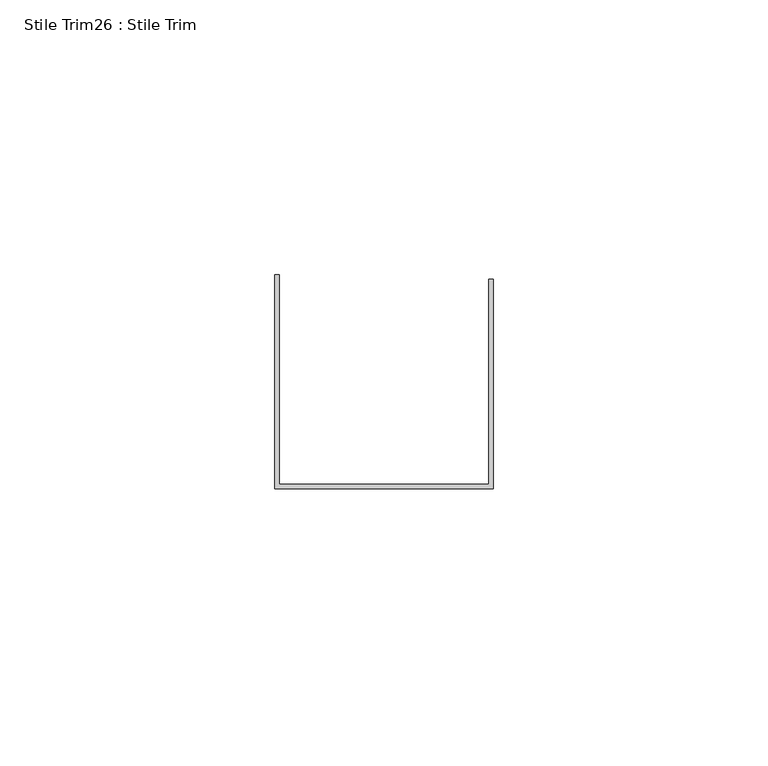
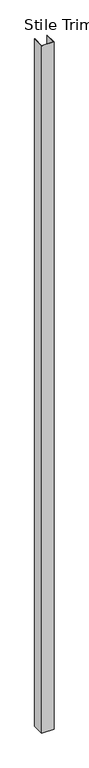
"""IFC4 building model written with IfcOpenShell, lengths in millimetres: proxy geometry, Stile Trim26 : Stile Trim."""

from ifc_helpers import new_model, si_unit, frame, origin, place, context, project, spatial, polyline, outline, extrude, source, transform, mapped, element, save


def stile_trim26_stile_trim_9ce5906b(model_context):
    return source(origin(), model_context, "Body", "SweptSolid", [
        extrude(outline(polyline([(587327.0060739, -536302.4912841), (587327.0060739, -536263.6038841), (587327.7934739, -536263.6038841), (587327.7934739, -536301.7038841), (587365.8934739, -536301.7038841), (587365.8934739, -536264.3912841), (587366.6808739, -536264.3912841), (587366.6808739, -536302.4912841), (587327.0060739, -536302.4912841)])), frame((0.0, 0.0, 50.8), z_axis=(0.0, 0.0, 1.0), x_axis=(1.0, 0.0, 0.0)), (0.0, 0.0, 1.0), 2350.3929688),
    ])


if __name__ == "__main__":
    model = new_model("IFC4")
    model_context = context("Model", 3, world=origin())
    ifc_project = project(units=[si_unit("LENGTHUNIT", "METRE", prefix="MILLI")], contexts=[model_context])
    site = spatial("IfcSite", under=ifc_project)
    building = spatial("IfcBuilding", under=site)
    placement = place(None, origin())
    stile_trim26_stile_trim_shape = stile_trim26_stile_trim_9ce5906b(model_context)
    element("IfcBuildingElementProxy", 1, Name="Stile Trim26 : Stile Trim", ObjectType="Stile Trim26 : Stile Trim", at=placement, inside=building, context=model_context, shape_type="MappedRepresentation", body=[
        mapped(stile_trim26_stile_trim_shape, transform((0.0, 0.0, 0.0), x_axis=(1.0, 0.0, 0.0), y_axis=(0.0, 1.0, 0.0), z_axis=(0.0, 0.0, 1.0))),
    ])
    save(model, "model.ifc")

# Revit data of these elements
# Element 1 (IfcBuildingElementProxy, "Stile Trim26 : Stile Trim")
#   Materials on its faces: "EDGE TRIM BY MTL PANEL MFR."
# Materials
#   "EDGE TRIM BY MTL PANEL MFR.": class "Generic", colour RGB 239 242 240, transparency 0, Cost = 0
